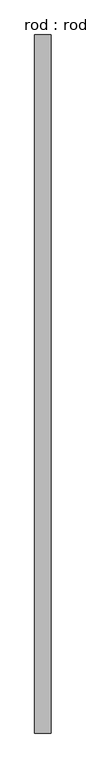
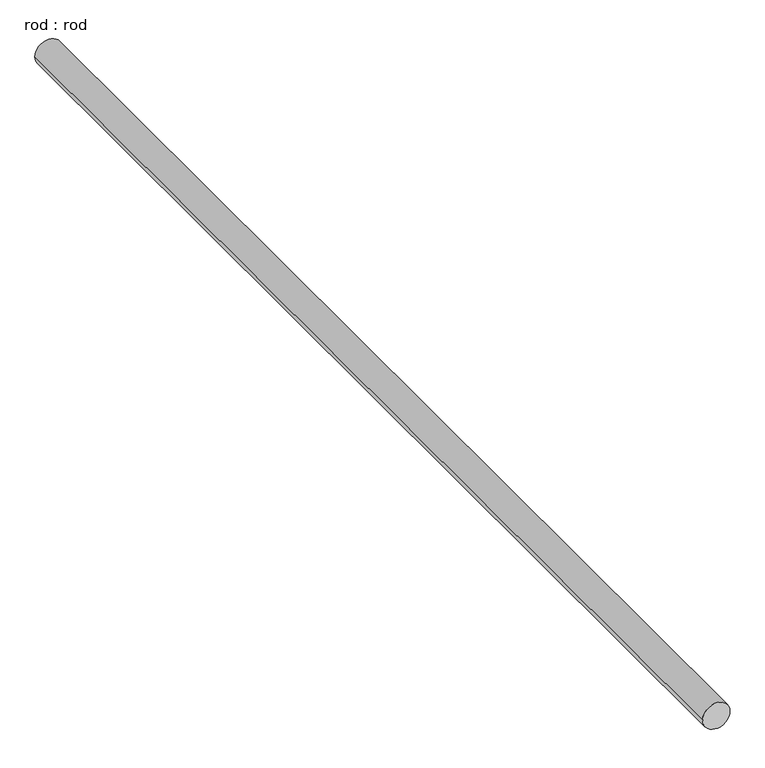
"""IFC4 building model written with IfcOpenShell, lengths in millimetres: proxy geometry, rod : rod."""

from ifc_helpers import new_model, si_unit, point, frame, frame_2d, origin, place, context, project, spatial, circle_curve, trimmed, segment, composite_curve, outline, extrude, source, transform, mapped, element, save


def rod_rod_fdba7ed2(model_context):
    return source(origin(), model_context, "Body", "SweptSolid", [
        extrude(outline(composite_curve([segment(trimmed(circle_curve(frame_2d((0.0108462, 0.0)), 200.0), [point((0.0108462, 200.0))], [point((0.0108462, -200.0))], False, "CARTESIAN"), True, "CONTINUOUS"), segment(trimmed(circle_curve(frame_2d((0.0108462, 0.0)), 200.0), [point((0.0108462, -200.0))], [point((0.0108462, 200.0))], False, "CARTESIAN"), True, "CONTINUOUS")], self_intersect=False)), frame((0.0, -4407.2713847, 0.0), z_axis=(0.0, 1.0, 0.0), x_axis=(0.0, 0.0, 1.0)), (0.0, 0.0, 1.0), 17000.0),
    ])


if __name__ == "__main__":
    model = new_model("IFC4")
    model_context = context("Model", 3, world=origin())
    ifc_project = project(units=[si_unit("LENGTHUNIT", "METRE", prefix="MILLI")], contexts=[model_context])
    site = spatial("IfcSite", under=ifc_project)
    building = spatial("IfcBuilding", under=site)
    placement = place(None, origin())
    rod_rod_shape = rod_rod_fdba7ed2(model_context)
    element("IfcBuildingElementProxy", 1, Name="rod : rod", ObjectType="rod : rod", at=placement, inside=building, context=model_context, shape_type="MappedRepresentation", body=[
        mapped(rod_rod_shape, transform((0.0, 0.0, 0.0), x_axis=(1.0, 0.0, 0.0), y_axis=(0.0, 1.0, 0.0), z_axis=(0.0, 0.0, 1.0))),
    ])
    save(model, "model.ifc")

# Revit data of these elements
# Type "rod : rod"
#   Default Elevation = 0
